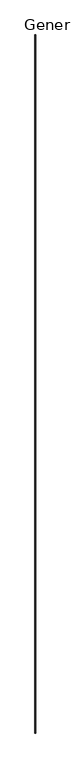
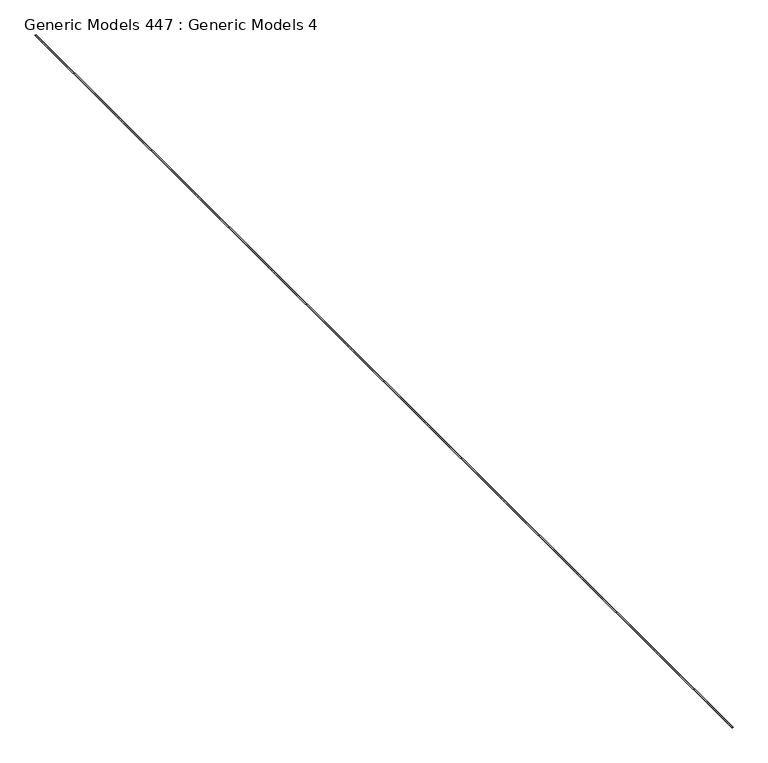
"""IFC4 building model written with IfcOpenShell, lengths in millimetres: proxy geometry, Generic Models 447 : Generic Models 4."""

from ifc_helpers import new_model, si_unit, point, frame, frame_2d, origin, place, context, project, spatial, polyline, circle_curve, trimmed, segment, composite_curve, outline, extrude, source, transform, mapped, element, save


def generic_models_447_generic_models_4_ea4d54c2(model_context):
    return source(origin(), model_context, "Body", "SweptSolid", [
        extrude(outline(composite_curve([segment(polyline([(126237.4210681, 1657.3182351), (126237.4210681, 1642.8008114)]), True, "CONTINUOUS"), segment(trimmed(circle_curve(frame_2d((126236.6273181, 1642.8008114)), 0.79375), [point((126237.4210681, 1642.8008114))], [point((126235.8335681, 1642.8008114))], False, "CARTESIAN"), True, "CONTINUOUS"), segment(polyline([(126235.8335681, 1642.8008114), (126235.8335681, 1657.3182351)]), True, "CONTINUOUS"), segment(trimmed(circle_curve(frame_2d((126236.6273181, 1657.3182351)), 0.79375), [point((126235.8335681, 1657.3182351))], [point((126237.4210681, 1657.3182351))], False, "CARTESIAN"), True, "CONTINUOUS")], self_intersect=False)), frame((0.0, -2064.0606022, 0.0), z_axis=(0.0, 1.0, 0.0), x_axis=(0.0, 0.0, 1.0)), (0.0, 0.0, 1.0), 13919.2),
    ])


if __name__ == "__main__":
    model = new_model("IFC4")
    model_context = context("Model", 3, world=origin())
    ifc_project = project(units=[si_unit("LENGTHUNIT", "METRE", prefix="MILLI")], contexts=[model_context])
    site = spatial("IfcSite", under=ifc_project)
    building = spatial("IfcBuilding", under=site)
    placement = place(None, origin())
    generic_models_447_generic_models_4_shape = generic_models_447_generic_models_4_ea4d54c2(model_context)
    element("IfcBuildingElementProxy", 1, Name="Generic Models 447 : Generic Models 4", ObjectType="Generic Models 447 : Generic Models 4", at=placement, inside=building, context=model_context, shape_type="MappedRepresentation", body=[
        mapped(generic_models_447_generic_models_4_shape, transform((0.0, 0.0, 0.0), x_axis=(1.0, 0.0, 0.0), y_axis=(0.0, 1.0, 0.0), z_axis=(0.0, 0.0, 1.0))),
    ])
    save(model, "model.ifc")

# Revit data of these elements
# Element 1 (IfcBuildingElementProxy, "Generic Models 447 : Generic Models 4")
#   Materials on its faces: "_BED OF SEALANT"
# Materials
#   "_BED OF SEALANT": class "Generic", colour RGB 253 192 103, transparency 0, Cost = 0
